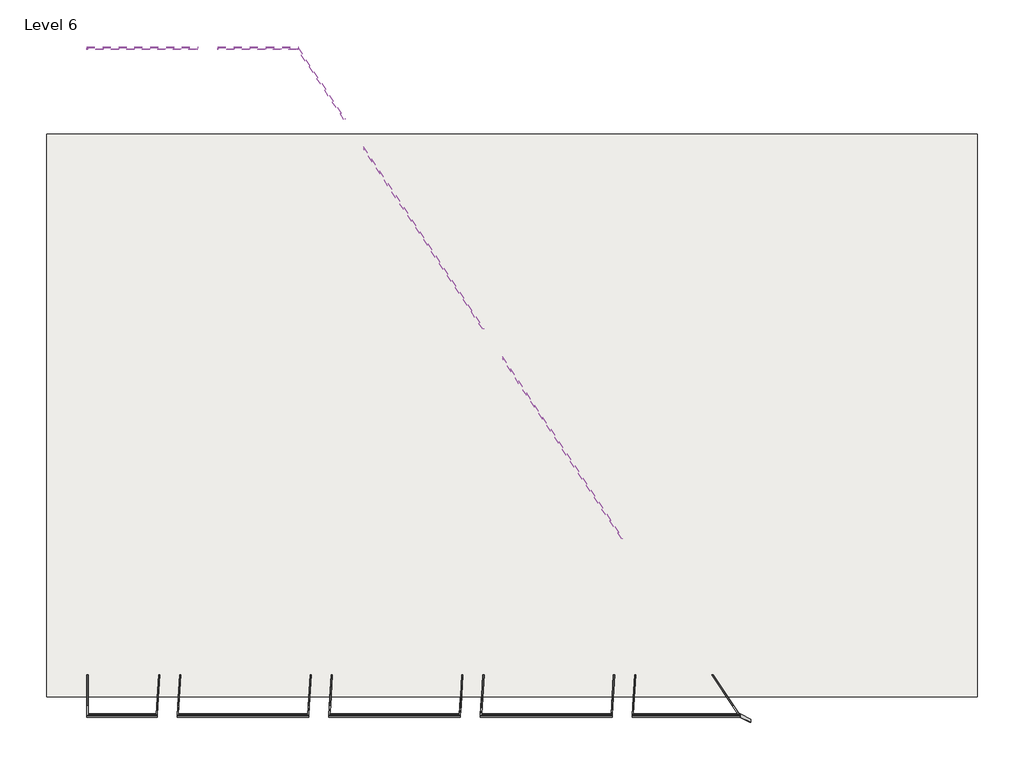
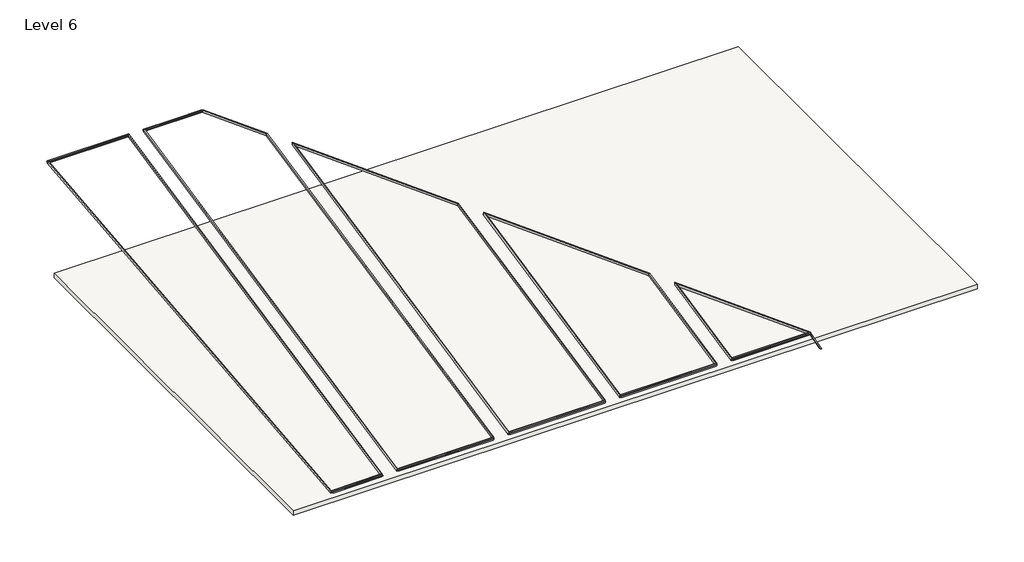
# One storey: 28 members, 1 slab.
"""IFC4 building model written with IfcOpenShell, lengths in millimetres."""

import ifcopenshell
import ifcopenshell.guid

model = None  # the IFC model being written
_history = None  # IfcOwnerHistory: only IFC2X3 demands one
_inside = {}  # id of a spatial element -> (the spatial element, [elements in it])
_under = {}  # id of a project, library or spatial element -> (it, [spatial elements below it])
_declared = {}  # id of a project -> (the project, [libraries it declares])
_typed = {}  # id of a type object -> (the type object, [elements of that type])
_made_of = {}  # id of a material, layer set ... -> (it, [elements and type objects made of it])


def new_model(schema):
    """Start an empty IFC model of exactly this schema.

    Asked for "IFC4X3", IfcOpenShell would pick the latest addendum, in which some entities
    have other attributes; the version numbers below select the first issue.
    IFC2X3 requires an IfcOwnerHistory on every rooted entity: one is made here for all.
    """
    global model, _history
    if schema == "IFC4X3":
        model = ifcopenshell.file(schema_version=(4, 3, 0, 0))
    else:
        model = ifcopenshell.file(schema=schema)
    _inside.clear()
    _under.clear()
    _declared.clear()
    _typed.clear()
    _made_of.clear()
    _history = None
    if model.schema == "IFC2X3":
        org = make("IfcOrganization", Name="unknown")
        user = make(
            "IfcPersonAndOrganization",
            ThePerson=make("IfcPerson", FamilyName="unknown"),
            TheOrganization=org,
        )
        app = make(
            "IfcApplication",
            ApplicationDeveloper=org,
            Version="unknown",
            ApplicationFullName="unknown",
            ApplicationIdentifier="unknown",
        )
        _history = make(
            "IfcOwnerHistory",
            OwningUser=user,
            OwningApplication=app,
            ChangeAction="ADDED",
            CreationDate=0,
        )
    return model


def make(cls, **values):
    """One entity of the class cls with the attributes given. An attribute that is None is left unset."""
    return model.create_entity(
        cls, **{name: value for name, value in values.items() if value is not None}
    )


def rooted(cls, **values):
    """An entity with a GlobalId (a new one), such as an element, a storey or a relation."""
    return make(cls, GlobalId=ifcopenshell.guid.new(), OwnerHistory=_history, **values)


def si_unit(unit_type, name, prefix=None):
    """IfcSIUnit, for example si_unit("LENGTHUNIT", "METRE", prefix="MILLI")."""
    return make("IfcSIUnit", UnitType=unit_type, Prefix=prefix, Name=name)


def assignment(units):
    """IfcUnitAssignment: the units of a project."""
    return None if units is None else make("IfcUnitAssignment", Units=units)


def point(xyz):
    """IfcCartesianPoint."""
    return None if xyz is None else make("IfcCartesianPoint", Coordinates=xyz)


def direction(xyz):
    """IfcDirection."""
    return None if xyz is None else make("IfcDirection", DirectionRatios=xyz)


def frame(location, z_axis=None, x_axis=None):
    """IfcAxis2Placement3D, a coordinate frame: its origin and axes. An axis left out is left unset."""
    return make(
        "IfcAxis2Placement3D",
        Location=point(location),
        Axis=direction(z_axis),
        RefDirection=direction(x_axis),
    )


def origin():
    """The frame at (0, 0, 0) with its axes left unset."""
    return frame((0.0, 0.0, 0.0))


def place(relative_to, where):
    """IfcLocalPlacement: puts the frame where relative to a parent placement (None: the world)."""
    return make(
        "IfcLocalPlacement", PlacementRelTo=relative_to, RelativePlacement=where
    )


def context(
    kind, dimensions, precision=None, world=None, true_north=None, identifier=None
):
    """IfcGeometricRepresentationContext, for example the 3D "Model" context."""
    return make(
        "IfcGeometricRepresentationContext",
        ContextIdentifier=identifier,
        ContextType=kind,
        CoordinateSpaceDimension=dimensions,
        Precision=precision,
        WorldCoordinateSystem=world,
        TrueNorth=true_north,
    )


def project(units=None, contexts=None):
    """IfcProject with its units and contexts."""
    return rooted(
        "IfcProject",
        Name="project",
        RepresentationContexts=contexts,
        UnitsInContext=assignment(units),
    )


def spatial(cls, under=None, at=None, **own):
    """A site, building, storey or space (cls), placed at a placement, below another one or the project."""
    s = rooted(cls, ObjectPlacement=at, **own)
    if under is not None:
        _under.setdefault(under.id(), (under, []))[1].append(s)
    return s


def polyline(points):
    """IfcPolyline through the points."""
    return make("IfcPolyline", Points=[point(p) for p in points])


def outline(outer, holes=None, kind="AREA"):
    """IfcArbitraryClosedProfileDef: a profile drawn as a closed curve; with holes, ...WithVoids."""
    if holes is None:
        return make("IfcArbitraryClosedProfileDef", ProfileType=kind, OuterCurve=outer)
    return make(
        "IfcArbitraryProfileDefWithVoids",
        ProfileType=kind,
        OuterCurve=outer,
        InnerCurves=holes,
    )


def extrude(swept, where, along, depth):
    """IfcExtrudedAreaSolid: the profile swept, set in the frame where, extruded along a direction by depth."""
    return make(
        "IfcExtrudedAreaSolid",
        SweptArea=swept,
        Position=where,
        ExtrudedDirection=direction(along),
        Depth=depth,
    )


def shape(context_of_items, identifier, shape_type, items):
    """IfcShapeRepresentation: the items that make up one representation, for example the "Body"."""
    return make(
        "IfcShapeRepresentation",
        ContextOfItems=context_of_items,
        RepresentationIdentifier=identifier,
        RepresentationType=shape_type,
        Items=items,
    )


def source(mapping_origin, context_of_items, identifier, shape_type, items):
    """IfcRepresentationMap: a shape defined once, which mapped items show again and again."""
    return make(
        "IfcRepresentationMap",
        MappingOrigin=mapping_origin,
        MappedRepresentation=shape(context_of_items, identifier, shape_type, items),
    )


def transform(
    local_origin,
    x_axis=None,
    y_axis=None,
    z_axis=None,
    scale=None,
    scale2=None,
    scale3=None,
    uniform=True,
):
    """IfcCartesianTransformationOperator3D, or its non-uniform kind. x_axis, y_axis, z_axis: its Axis1, 2, 3."""
    if uniform:
        return make(
            "IfcCartesianTransformationOperator3D",
            Axis1=direction(x_axis),
            Axis2=direction(y_axis),
            LocalOrigin=point(local_origin),
            Scale=scale,
            Axis3=direction(z_axis),
        )
    return make(
        "IfcCartesianTransformationOperator3DnonUniform",
        Axis1=direction(x_axis),
        Axis2=direction(y_axis),
        LocalOrigin=point(local_origin),
        Scale=scale,
        Axis3=direction(z_axis),
        Scale2=scale2,
        Scale3=scale3,
    )


def mapped(mapping_source, mapping_target):
    """IfcMappedItem: shows the shape of a source again, moved by a transform."""
    return make(
        "IfcMappedItem", MappingSource=mapping_source, MappingTarget=mapping_target
    )


def made_of(thing, what):
    """Note that an element or type object is made of a material, layer set ...; save() writes the relation."""
    if what is not None:
        _made_of.setdefault(what.id(), (what, []))[1].append(thing)
    return thing


def element(
    cls,
    number,
    at=None,
    inside=None,
    cuts=None,
    type_object=None,
    material=None,
    context=None,
    identifier="Body",
    shape_type=None,
    held_by="IfcProductDefinitionShape",
    body=None,
    shapes=None,
    **own,
):
    """One element of the class cls, such as IfcWall. Its Tag is "e" and its number.

    at: its placement. inside: the storey or other place that contains it. cuts: it is an
    opening in that element (IfcRelVoidsElement). A single representation is given by context,
    identifier, shape_type and body (its items); several are given by shapes. held_by: the class
    of the entity that holds the representations. save() writes the other relations.
    """
    e = rooted(cls, Tag="e%d" % number, ObjectPlacement=at, **own)
    if body is not None:
        shapes = [shape(context, identifier, shape_type, body)]
    if shapes is not None:
        e.Representation = make(held_by, Representations=shapes)
    if inside is not None:
        _inside.setdefault(inside.id(), (inside, []))[1].append(e)
    if cuts is not None:
        rooted(
            "IfcRelVoidsElement", RelatingBuildingElement=cuts, RelatedOpeningElement=e
        )
    if type_object is not None:
        _typed.setdefault(type_object.id(), (type_object, []))[1].append(e)
    return made_of(e, material)


def aggregate(whole, parts):
    """IfcRelAggregates: a whole, such as a stair, and the parts it consists of."""
    return rooted("IfcRelAggregates", RelatingObject=whole, RelatedObjects=parts)


def save(model, path):
    """Write the relations noted so far, then the file.

    IfcRelAggregates (storeys below a building ...), IfcRelContainedInSpatialStructure (elements
    in a storey), IfcRelDefinesByType, IfcRelAssociatesMaterial and IfcRelDeclares: one each for
    every whole, place, type object, material and project.
    """
    for whole, parts in _under.values():
        aggregate(whole, parts)
    for where, things in _inside.values():
        rooted(
            "IfcRelContainedInSpatialStructure",
            RelatedElements=things,
            RelatingStructure=where,
        )
    for kind, things in _typed.values():
        rooted("IfcRelDefinesByType", RelatedObjects=things, RelatingType=kind)
    for what, things in _made_of.values():
        rooted("IfcRelAssociatesMaterial", RelatedObjects=things, RelatingMaterial=what)
    for by, libraries in _declared.values():
        rooted("IfcRelDeclares", RelatingContext=by, RelatedDefinitions=libraries)
    model.write(path)


def rectangular_mullion_50_x_150mm_a1f019ed(model_context):
    return source(origin(), model_context, "Body", "SweptSolid", [
        extrude(outline(polyline([(0.0, 0.0), (-58.5251446, -50.0), (-1143.6098029, -50.0), (-1169.4475431, 0.0), (0.0, 0.0)])), frame((0.0, -75.0, 0.0), z_axis=(0.0, 1.0, 0.0), x_axis=(0.0, 0.0, 1.0)), (0.0, 0.0, 1.0), 150.0),
    ])


def rectangular_mullion_50_x_150mm_835307d9(model_context):
    return source(origin(), model_context, "Body", "SweptSolid", [
        extrude(outline(polyline([(0.0, 0.0), (-53.1084457, -50.0), (-6798.2667293, -50.0), (-6948.5596255, 0.0), (0.0, 0.0)])), frame((0.0, -75.0, 0.0), z_axis=(0.0, 1.0, 0.0), x_axis=(0.0, 0.0, 1.0)), (0.0, 0.0, 1.0), 150.0),
    ])


def rectangular_mullion_50_x_150mm_3a89df96(model_context):
    return source(origin(), model_context, "Body", "SweptSolid", [
        extrude(outline(polyline([(0.0, 0.0), (-50.0, -50.0), (-30950.0, -50.0), (-31000.0, 0.0), (0.0, 0.0)])), frame((0.0, -75.0, 0.0), z_axis=(0.0, 1.0, 0.0), x_axis=(0.0, 0.0, 1.0)), (0.0, 0.0, 1.0), 150.0),
    ])


def rectangular_mullion_50_x_150mm_0c0d54b6(model_context):
    return source(origin(), model_context, "Body", "SweptSolid", [
        extrude(outline(polyline([(0.0, 0.0), (-53.1084457, -50.0), (-31009.3272322, -50.0), (-31056.4007243, 0.0), (0.0, 0.0)])), frame((0.0, -75.0, 0.0), z_axis=(0.0, 1.0, 0.0), x_axis=(0.0, 0.0, 1.0)), (0.0, 0.0, 1.0), 150.0),
    ])


def rectangular_mullion_50_x_150mm_d5752ba3(model_context):
    return source(origin(), model_context, "Body", "SweptSolid", [
        extrude(outline(polyline([(0.0, 0.0), (-53.1084457, -50.0), (-26319.8624924, -50.0), (-26470.1553886, 0.0), (0.0, 0.0)])), frame((0.0, -75.0, 0.0), z_axis=(0.0, 1.0, 0.0), x_axis=(0.0, 0.0, 1.0)), (0.0, 0.0, 1.0), 150.0),
    ])


def rectangular_mullion_50_x_150mm_d02c79f9(model_context):
    return source(origin(), model_context, "Body", "SweptSolid", [
        extrude(outline(polyline([(0.0, 0.0), (-53.1084457, -50.0), (-16559.0646109, -50.0), (-16709.3575071, 0.0), (0.0, 0.0)])), frame((0.0, -75.0, 0.0), z_axis=(0.0, 1.0, 0.0), x_axis=(0.0, 0.0, 1.0)), (0.0, 0.0, 1.0), 150.0),
    ])


def rectangular_mullion_50_x_150mm_9a9dcb3f(model_context):
    return source(origin(), model_context, "Body", "SweptSolid", [
        extrude(outline(polyline([(0.0, 0.0), (-150.2928962, -50.0), (-8210.4264863, -50.0), (-8303.1882256, 0.0), (0.0, 0.0)])), frame((0.0, -75.0, 0.0), z_axis=(0.0, 1.0, 0.0), x_axis=(0.0, 0.0, 1.0)), (0.0, 0.0, 1.0), 150.0),
    ])


def rectangular_mullion_50_x_150mm_8c2aeeaa(model_context):
    return source(origin(), model_context, "Body", "SweptSolid", [
        extrude(outline(polyline([(0.0, 0.0), (-26.9507667, -50.0), (-3926.5430895, -50.0), (-3943.1772756, 0.0), (0.0, 0.0)])), frame((0.0, -75.0, 0.0), z_axis=(0.0, 1.0, 0.0), x_axis=(0.0, 0.0, 1.0)), (0.0, 0.0, 1.0), 150.0),
    ])


def rectangular_mullion_50_x_150mm_b203450d(model_context):
    return source(origin(), model_context, "Body", "SweptSolid", [
        extrude(outline(polyline([(0.0, 0.0), (-16.6341861, -50.0), (-27709.4619673, -50.0), (-27756.5354594, 0.0), (0.0, 0.0)])), frame((0.0, -75.0, 0.0), z_axis=(0.0, 1.0, 0.0), x_axis=(0.0, 0.0, 1.0)), (0.0, 0.0, 1.0), 150.0),
    ])


def rectangular_mullion_50_x_150mm_36cf8f86(model_context):
    return source(origin(), model_context, "Body", "SweptSolid", [
        extrude(outline(polyline([(0.0, 0.0), (-150.2928962, -50.0), (-10109.8797934, -50.0), (-10126.5139795, 0.0), (0.0, 0.0)])), frame((0.0, -75.0, 0.0), z_axis=(0.0, 1.0, 0.0), x_axis=(0.0, 0.0, 1.0)), (0.0, 0.0, 1.0), 150.0),
    ])


def rectangular_mullion_50_x_150mm_3d894c4c(model_context):
    return source(origin(), model_context, "Body", "SweptSolid", [
        extrude(outline(polyline([(0.0, 0.0), (-16.6341861, -50.0), (-17948.6640858, -50.0), (-17995.7375779, 0.0), (0.0, 0.0)])), frame((0.0, -75.0, 0.0), z_axis=(0.0, 1.0, 0.0), x_axis=(0.0, 0.0, 1.0)), (0.0, 0.0, 1.0), 150.0),
    ])


def rectangular_mullion_50_x_150mm_f4970be0(model_context):
    return source(origin(), model_context, "Body", "SweptSolid", [
        extrude(outline(polyline([(0.0, 0.0), (-16.6341861, -50.0), (-8187.8662042, -50.0), (-8234.9396963, 0.0), (0.0, 0.0)])), frame((0.0, -75.0, 0.0), z_axis=(0.0, 1.0, 0.0), x_axis=(0.0, 0.0, 1.0)), (0.0, 0.0, 1.0), 150.0),
    ])


def rectangular_mullion_50_x_150mm_5700b0c8(model_context):
    return source(origin(), model_context, "Body", "SweptSolid", [
        extrude(outline(polyline([(0.0, 0.0), (-86.4378444, -50.0), (-5081.8724884, -50.0), (-5115.611673, 0.0), (0.0, 0.0)])), frame((0.0, -75.0, 0.0), z_axis=(0.0, 1.0, 0.0), x_axis=(0.0, 0.0, 1.0)), (0.0, 0.0, 1.0), 150.0),
    ])


def rectangular_mullion_50_x_150mm_c12f4f4b(model_context):
    return source(origin(), model_context, "Body", "SweptSolid", [
        extrude(outline(polyline([(0.0, 0.0), (-98.1080667, -50.0), (-3682.0310611, -50.0), (-3710.9535778, 0.0), (0.0, 0.0)])), frame((0.0, -75.0, 0.0), z_axis=(0.0, 1.0, 0.0), x_axis=(0.0, 0.0, 1.0)), (0.0, 0.0, 1.0), 150.0),
    ])


def rectangular_mullion_50_x_150mm_5a0cd9cb(model_context):
    return source(origin(), model_context, "Body", "SweptSolid", [
        extrude(outline(polyline([(0.0, 0.0), (-92.7617394, -50.0), (-4930.0822697, -50.0), (-4983.1907154, 0.0), (0.0, 0.0)])), frame((0.0, -75.0, 0.0), z_axis=(0.0, 1.0, 0.0), x_axis=(0.0, 0.0, 1.0)), (0.0, 0.0, 1.0), 150.0),
    ])


def rectangular_mullion_50_x_150mm_5afc71bb(model_context):
    return source(origin(), model_context, "Body", "SweptSolid", [
        extrude(outline(polyline([(0.0, 0.0), (-47.0734921, -50.0), (-3194.7760444, -50.0), (-3244.7760444, 0.0), (0.0, 0.0)])), frame((0.0, -75.0, 0.0), z_axis=(0.0, 1.0, 0.0), x_axis=(0.0, 0.0, 1.0)), (0.0, 0.0, 1.0), 150.0),
    ])


def rectangular_mullion_50_x_150mm_f23ada83(model_context):
    return source(origin(), model_context, "Body", "SweptSolid", [
        extrude(outline(polyline([(0.0, 0.0), (-47.0734921, -50.0), (-6024.3583142, -50.0), (-6077.4667599, 0.0), (0.0, 0.0)])), frame((0.0, -75.0, 0.0), z_axis=(0.0, 1.0, 0.0), x_axis=(0.0, 0.0, 1.0)), (0.0, 0.0, 1.0), 150.0),
    ])


def rectangular_mullion_50_x_150mm_0be3d6d3(model_context):
    return source(origin(), model_context, "Body", "SweptSolid", [
        extrude(outline(polyline([(0.0, 0.0), (-50.0, -50.0), (-5062.5032273, -50.0), (-5115.611673, 0.0), (0.0, 0.0)])), frame((0.0, -75.0, 0.0), z_axis=(0.0, 1.0, 0.0), x_axis=(0.0, 0.0, 1.0)), (0.0, 0.0, 1.0), 150.0),
    ])


def rectangular_mullion_50_x_150mm_139992b9(model_context):
    return source(origin(), model_context, "Body", "SweptSolid", [
        extrude(outline(polyline([(0.0, 0.0), (-47.0734921, -50.0), (-3684.0028111, -50.0), (-3710.9535778, 0.0), (0.0, 0.0)])), frame((0.0, -75.0, 0.0), z_axis=(0.0, 1.0, 0.0), x_axis=(0.0, 0.0, 1.0)), (0.0, 0.0, 1.0), 150.0),
    ])


def rectangular_mullion_50_x_150mm_45cfd48e(model_context):
    return source(origin(), model_context, "Body", "SweptSolid", [
        extrude(outline(polyline([(0.0, 0.0), (-108.6604448, -50.0), (-3159.4549255, -50.0), (-3244.7760444, 0.0), (0.0, 0.0)])), frame((0.0, -75.0, 0.0), z_axis=(0.0, 1.0, 0.0), x_axis=(0.0, 0.0, 1.0)), (0.0, 0.0, 1.0), 150.0),
    ])


def rectangular_mullion_50_x_150mm_f412d67c(model_context):
    return source(origin(), model_context, "Body", "SweptSolid", [
        extrude(outline(polyline([(0.0, 0.0), (-29.3010691, -50.0), (-5992.1456409, -50.0), (-6077.4667599, 0.0), (0.0, 0.0)])), frame((0.0, -75.0, 0.0), z_axis=(0.0, 1.0, 0.0), x_axis=(0.0, 0.0, 1.0)), (0.0, 0.0, 1.0), 150.0),
    ])


def rectangular_mullion_50_x_150mm_460fb724(model_context):
    return source(origin(), model_context, "Body", "SweptSolid", [
        extrude(outline(polyline([(0.0, 0.0), (-29.3010691, -50.0), (-4821.4590794, -50.0), (-4983.1907154, 0.0), (0.0, 0.0)])), frame((0.0, -75.0, 0.0), z_axis=(0.0, 1.0, 0.0), x_axis=(0.0, 0.0, 1.0)), (0.0, 0.0, 1.0), 150.0),
    ])


model = new_model("IFC4")

# Units and contexts
model_context = context("Model", 3, world=origin())
ifc_project = project(units=[si_unit("LENGTHUNIT", "METRE", prefix="MILLI")], contexts=[model_context])

# Site, building, storey
site = spatial("IfcSite", under=ifc_project)
building = spatial("IfcBuilding", under=site)
storey = spatial("IfcBuildingStorey", under=building, Name="Level 6", Elevation=15000.0)

# Members
placement = place(None, origin())
rectangular_mullion_50_x_150mm_shape = rectangular_mullion_50_x_150mm_a1f019ed(model_context)
element("IfcMember", 1, ObjectType="Rectangular Mullion : 50 x 150mm", at=placement, inside=storey, context=model_context, shape_type="MappedRepresentation", body=[
    mapped(rectangular_mullion_50_x_150mm_shape, transform((25283.6081085, -10856.2576342, 16077.9460567), x_axis=(0.9035184763618896, 0.10483186655429763, 0.41552935230550386), y_axis=(-0.004309282844983733, 0.9717923608297843, -0.23579872246099295), z_axis=(-0.42852747047774137, 0.2112578689365591, 0.8784841033612003))),
])
rectangular_mullion_50_x_150mm_2_shape = rectangular_mullion_50_x_150mm_835307d9(model_context)
element("IfcMember", 2, ObjectType="Rectangular Mullion : 50 x 150mm", at=placement, inside=storey, context=model_context, shape_type="MappedRepresentation", body=[
    mapped(rectangular_mullion_50_x_150mm_2_shape, transform((20300.417393, -10856.2576342, 16077.9460567), x_axis=(-0.9981839259219352, 0.05990993649800364, 0.006296788060437585), y_axis=(0.0, 0.10452846326765378, -0.9945218953682734), z_axis=(-0.06023993717686712, -0.9927157699340269, -0.10433863183509343))),
])
rectangular_mullion_50_x_150mm_3_shape = rectangular_mullion_50_x_150mm_3a89df96(model_context)
element("IfcMember", 3, ObjectType="Rectangular Mullion : 50 x 150mm", at=placement, inside=storey, context=model_context, shape_type="MappedRepresentation", body=[
    mapped(rectangular_mullion_50_x_150mm_3_shape, transform((-4866.8918915, -10856.2576342, 16077.9460567), x_axis=(-1.0, 0.0, 0.0), y_axis=(0.0, 0.10452846326765393, -0.9945218953682733), z_axis=(0.0, -0.9945218953682733, -0.10452846326765393))),
])
rectangular_mullion_50_x_150mm_4_shape = rectangular_mullion_50_x_150mm_0c0d54b6(model_context)
element("IfcMember", 4, ObjectType="Rectangular Mullion : 50 x 150mm", at=placement, inside=storey, context=model_context, shape_type="MappedRepresentation", body=[
    mapped(rectangular_mullion_50_x_150mm_4_shape, transform((-699.582607, -10856.2576342, 16077.9460567), x_axis=(-0.998183925921935, 0.05990993649800494, 0.00629678806043772), y_axis=(0.0, 0.10452846326765394, -0.9945218953682733), z_axis=(-0.06023993717686844, -0.9927157699340269, -0.1043386318350936))),
])
rectangular_mullion_50_x_150mm_5_shape = rectangular_mullion_50_x_150mm_d5752ba3(model_context)
element("IfcMember", 5, ObjectType="Rectangular Mullion : 50 x 150mm", at=placement, inside=storey, context=model_context, shape_type="MappedRepresentation", body=[
    mapped(rectangular_mullion_50_x_150mm_5_shape, transform((6300.417393, -10856.2576342, 16077.9460567), x_axis=(-0.9981839259219351, 0.059909936498005, 0.006296788060437727), y_axis=(0.0, 0.10452846326765393, -0.9945218953682734), z_axis=(-0.060239937176868485, -0.9927157699340268, -0.10433863183509358))),
])
rectangular_mullion_50_x_150mm_6_shape = rectangular_mullion_50_x_150mm_d02c79f9(model_context)
element("IfcMember", 6, ObjectType="Rectangular Mullion : 50 x 150mm", at=placement, inside=storey, context=model_context, shape_type="MappedRepresentation", body=[
    mapped(rectangular_mullion_50_x_150mm_6_shape, transform((13300.417393, -10856.2576342, 16077.9460567), x_axis=(-0.998183925921935, 0.05990993649800466, 0.006296788060437691), y_axis=(0.0, 0.1045284632676539, -0.9945218953682733), z_axis=(-0.06023993717686815, -0.9927157699340269, -0.10433863183509358))),
])
rectangular_mullion_50_x_150mm_7_shape = rectangular_mullion_50_x_150mm_9a9dcb3f(model_context)
element("IfcMember", 7, ObjectType="Rectangular Mullion : 50 x 150mm", at=placement, inside=storey, context=model_context, shape_type="MappedRepresentation", body=[
    mapped(rectangular_mullion_50_x_150mm_7_shape, transform((20718.9981883, -3958.3129157, 16802.9492613), x_axis=(0.83533461340766, 0.5467302903451189, 0.05746366906330552), y_axis=(0.0, 0.10452846326765378, -0.9945218953682733), z_axis=(-0.5497418336301824, 0.83075856299291, 0.08731624345378214))),
])
element("IfcMember", 8, ObjectType="Rectangular Mullion : 50 x 150mm", at=placement, inside=storey, context=model_context, shape_type="MappedRepresentation", body=[
    mapped(rectangular_mullion_50_x_150mm_4_shape, transform((248.7197815, 19973.9211222, 19318.328418), x_axis=(0.998183925921935, -0.05990993649800525, -0.006296788060437753), y_axis=(0.0, 0.10452846326765385, -0.9945218953682734), z_axis=(0.06023993717686875, 0.9927157699340269, 0.10433863183509351))),
])
rectangular_mullion_50_x_150mm_8_shape = rectangular_mullion_50_x_150mm_8c2aeeaa(model_context)
element("IfcMember", 9, ObjectType="Rectangular Mullion : 50 x 150mm", at=placement, inside=storey, context=model_context, shape_type="MappedRepresentation", body=[
    mapped(rectangular_mullion_50_x_150mm_8_shape, transform((4882.2065994, 19973.9211222, 19318.328418), x_axis=(0.8353346134076604, 0.5467302903451184, 0.05746366906330546), y_axis=(0.0, 0.10452846326765367, -0.9945218953682733), z_axis=(-0.5497418336301818, 0.8307585629929103, 0.08731624345378203))),
])
rectangular_mullion_50_x_150mm_9_shape = rectangular_mullion_50_x_150mm_b203450d(model_context)
element("IfcMember", 10, ObjectType="Rectangular Mullion : 50 x 150mm", at=placement, inside=storey, context=model_context, shape_type="MappedRepresentation", body=[
    mapped(rectangular_mullion_50_x_150mm_9_shape, transform((7049.9361052, 16698.0928351, 18974.024991), x_axis=(0.998183925921935, -0.05990993649800497, -0.006296788060437724), y_axis=(0.0, 0.10452846326765391, -0.9945218953682734), z_axis=(0.060239937176868465, 0.9927157699340269, 0.10433863183509358))),
])
rectangular_mullion_50_x_150mm_10_shape = rectangular_mullion_50_x_150mm_36cf8f86(model_context)
element("IfcMember", 11, ObjectType="Rectangular Mullion : 50 x 150mm", at=placement, inside=storey, context=model_context, shape_type="MappedRepresentation", body=[
    mapped(rectangular_mullion_50_x_150mm_10_shape, transform((7894.9778907, 15421.0830526, 18839.8058544), x_axis=(0.83533461340766, 0.546730290345119, 0.05746366906330553), y_axis=(0.0, 0.10452846326765391, -0.9945218953682733), z_axis=(-0.5497418336301826, 0.83075856299291, 0.0873162434537823))),
])
rectangular_mullion_50_x_150mm_11_shape = rectangular_mullion_50_x_150mm_3d894c4c(model_context)
element("IfcMember", 12, ObjectType="Rectangular Mullion : 50 x 150mm", at=placement, inside=storey, context=model_context, shape_type="MappedRepresentation", body=[
    mapped(rectangular_mullion_50_x_150mm_11_shape, transform((13461.946254, 7008.3948509, 17955.5966945), x_axis=(0.9981839259219351, -0.05990993649800527, -0.006296788060437756), y_axis=(0.0, 0.10452846326765394, -0.9945218953682734), z_axis=(0.060239937176868756, 0.9927157699340268, 0.10433863183509359))),
])
element("IfcMember", 13, ObjectType="Rectangular Mullion : 50 x 150mm", at=placement, inside=storey, context=model_context, shape_type="MappedRepresentation", body=[
    mapped(rectangular_mullion_50_x_150mm_10_shape, transform((14306.9880395, 5731.3850685, 17821.3775579), x_axis=(0.8353346134076599, 0.5467302903451192, 0.05746366906330556), y_axis=(0.0, 0.10452846326765397, -0.9945218953682733), z_axis=(-0.5497418336301827, 0.8307585629929097, 0.08731624345378232))),
])
rectangular_mullion_50_x_150mm_12_shape = rectangular_mullion_50_x_150mm_f4970be0(model_context)
element("IfcMember", 14, ObjectType="Rectangular Mullion : 50 x 150mm", at=placement, inside=storey, context=model_context, shape_type="MappedRepresentation", body=[
    mapped(rectangular_mullion_50_x_150mm_12_shape, transform((19873.9564029, -2681.3031332, 16937.1683979), x_axis=(0.9981839259219351, -0.05990993649800277, -0.006296788060437492), y_axis=(0.0, 0.10452846326765383, -0.9945218953682733), z_axis=(0.06023993717686625, 0.992715769934027, 0.10433863183509351))),
])
rectangular_mullion_50_x_150mm_13_shape = rectangular_mullion_50_x_150mm_5700b0c8(model_context)
element("IfcMember", 15, ObjectType="Rectangular Mullion : 50 x 150mm", at=placement, inside=storey, context=model_context, shape_type="MappedRepresentation", body=[
    mapped(rectangular_mullion_50_x_150mm_13_shape, transform((248.7197815, 19973.9211222, 19318.328418), x_axis=(0.0, 0.08715574274766863, 0.9961946980917447), y_axis=(0.0, -0.9961946980917447, 0.08715574274766863), z_axis=(1.0, 0.0, 0.0))),
])
rectangular_mullion_50_x_150mm_14_shape = rectangular_mullion_50_x_150mm_c12f4f4b(model_context)
element("IfcMember", 16, ObjectType="Rectangular Mullion : 50 x 150mm", at=placement, inside=storey, context=model_context, shape_type="MappedRepresentation", body=[
    mapped(rectangular_mullion_50_x_150mm_14_shape, transform((4882.2065994, 19973.9211222, 19318.328418), x_axis=(0.0, 0.08715574274766863, 0.9961946980917447), y_axis=(0.0, -0.9961946980917447, 0.08715574274766863), z_axis=(1.0, 0.0, 0.0))),
])
rectangular_mullion_50_x_150mm_15_shape = rectangular_mullion_50_x_150mm_5a0cd9cb(model_context)
element("IfcMember", 17, ObjectType="Rectangular Mullion : 50 x 150mm", at=placement, inside=storey, context=model_context, shape_type="MappedRepresentation", body=[
    mapped(rectangular_mullion_50_x_150mm_15_shape, transform((25283.6081085, -10856.2576342, 16077.9460567), x_axis=(0.0, -0.9945218953682733, -0.10452846326765391), y_axis=(0.0, 0.10452846326765391, -0.9945218953682733), z_axis=(1.0, 0.0, 0.0))),
])
rectangular_mullion_50_x_150mm_16_shape = rectangular_mullion_50_x_150mm_5afc71bb(model_context)
element("IfcMember", 18, ObjectType="Rectangular Mullion : 50 x 150mm", at=placement, inside=storey, context=model_context, shape_type="MappedRepresentation", body=[
    mapped(rectangular_mullion_50_x_150mm_16_shape, transform((-1622.1158471, -10856.2576342, 16077.9460567), x_axis=(0.0, -0.9945218953682733, -0.10452846326765391), y_axis=(0.0, 0.10452846326765391, -0.9945218953682733), z_axis=(1.0, 0.0, 0.0))),
])
rectangular_mullion_50_x_150mm_17_shape = rectangular_mullion_50_x_150mm_f23ada83(model_context)
element("IfcMember", 19, ObjectType="Rectangular Mullion : 50 x 150mm", at=placement, inside=storey, context=model_context, shape_type="MappedRepresentation", body=[
    mapped(rectangular_mullion_50_x_150mm_17_shape, transform((5377.8841529, -10856.2576342, 16077.9460567), x_axis=(0.0, -0.9945218953682733, -0.10452846326765391), y_axis=(0.0, 0.10452846326765391, -0.9945218953682733), z_axis=(1.0, 0.0, 0.0))),
])
element("IfcMember", 20, ObjectType="Rectangular Mullion : 50 x 150mm", at=placement, inside=storey, context=model_context, shape_type="MappedRepresentation", body=[
    mapped(rectangular_mullion_50_x_150mm_17_shape, transform((12377.8841529, -10856.2576342, 16077.9460567), x_axis=(0.0, -0.9945218953682733, -0.10452846326765391), y_axis=(0.0, 0.10452846326765391, -0.9945218953682733), z_axis=(1.0, 0.0, 0.0))),
])
element("IfcMember", 21, ObjectType="Rectangular Mullion : 50 x 150mm", at=placement, inside=storey, context=model_context, shape_type="MappedRepresentation", body=[
    mapped(rectangular_mullion_50_x_150mm_17_shape, transform((19377.8841529, -10856.2576342, 16077.9460567), x_axis=(0.0, -0.9945218953682733, -0.10452846326765391), y_axis=(0.0, 0.10452846326765391, -0.9945218953682733), z_axis=(1.0, 0.0, 0.0))),
])
rectangular_mullion_50_x_150mm_18_shape = rectangular_mullion_50_x_150mm_0be3d6d3(model_context)
element("IfcMember", 22, ObjectType="Rectangular Mullion : 50 x 150mm", at=placement, inside=storey, context=model_context, shape_type="MappedRepresentation", body=[
    mapped(rectangular_mullion_50_x_150mm_18_shape, transform((-4866.8918915, 19973.9211222, 19318.328418), x_axis=(0.0, 0.9945218953682733, 0.10452846326765391), y_axis=(0.0, 0.10452846326765391, -0.9945218953682733), z_axis=(-1.0, 0.0, 0.0))),
])
rectangular_mullion_50_x_150mm_19_shape = rectangular_mullion_50_x_150mm_139992b9(model_context)
element("IfcMember", 23, ObjectType="Rectangular Mullion : 50 x 150mm", at=placement, inside=storey, context=model_context, shape_type="MappedRepresentation", body=[
    mapped(rectangular_mullion_50_x_150mm_19_shape, transform((1171.2530216, 19973.9211222, 19318.328418), x_axis=(0.0, 0.9945218953682733, 0.10452846326765391), y_axis=(0.0, 0.10452846326765391, -0.9945218953682733), z_axis=(-1.0, 0.0, 0.0))),
])
rectangular_mullion_50_x_150mm_20_shape = rectangular_mullion_50_x_150mm_45cfd48e(model_context)
element("IfcMember", 24, ObjectType="Rectangular Mullion : 50 x 150mm", at=placement, inside=storey, context=model_context, shape_type="MappedRepresentation", body=[
    mapped(rectangular_mullion_50_x_150mm_20_shape, transform((-4866.8918915, -10856.2576342, 16077.9460567), x_axis=(0.0, 0.24192189559966848, 0.9702957262759964), y_axis=(0.0, 0.9702957262759964, -0.24192189559966848), z_axis=(-1.0, 0.0, 0.0))),
])
rectangular_mullion_50_x_150mm_21_shape = rectangular_mullion_50_x_150mm_f412d67c(model_context)
element("IfcMember", 25, ObjectType="Rectangular Mullion : 50 x 150mm", at=placement, inside=storey, context=model_context, shape_type="MappedRepresentation", body=[
    mapped(rectangular_mullion_50_x_150mm_21_shape, transform((-699.582607, -10856.2576342, 16077.9460567), x_axis=(0.0, 0.24192189559966848, 0.9702957262759964), y_axis=(0.0, 0.9702957262759964, -0.24192189559966848), z_axis=(-1.0, 0.0, 0.0))),
])
element("IfcMember", 26, ObjectType="Rectangular Mullion : 50 x 150mm", at=placement, inside=storey, context=model_context, shape_type="MappedRepresentation", body=[
    mapped(rectangular_mullion_50_x_150mm_21_shape, transform((6300.417393, -10856.2576342, 16077.9460567), x_axis=(0.0, 0.24192189559966848, 0.9702957262759964), y_axis=(0.0, 0.9702957262759964, -0.24192189559966848), z_axis=(-1.0, 0.0, 0.0))),
])
element("IfcMember", 27, ObjectType="Rectangular Mullion : 50 x 150mm", at=placement, inside=storey, context=model_context, shape_type="MappedRepresentation", body=[
    mapped(rectangular_mullion_50_x_150mm_21_shape, transform((13300.417393, -10856.2576342, 16077.9460567), x_axis=(0.0, 0.24192189559966848, 0.9702957262759964), y_axis=(0.0, 0.9702957262759964, -0.24192189559966848), z_axis=(-1.0, 0.0, 0.0))),
])
rectangular_mullion_50_x_150mm_22_shape = rectangular_mullion_50_x_150mm_460fb724(model_context)
element("IfcMember", 28, ObjectType="Rectangular Mullion : 50 x 150mm", at=placement, inside=storey, context=model_context, shape_type="MappedRepresentation", body=[
    mapped(rectangular_mullion_50_x_150mm_22_shape, transform((20300.417393, -10856.2576342, 16077.9460567), x_axis=(0.0, 0.24192189559966848, 0.9702957262759964), y_axis=(0.0, 0.9702957262759964, -0.24192189559966848), z_axis=(-1.0, 0.0, 0.0))),
])

# Slab
element("IfcSlab", 29, ObjectType="Generic 300mm", at=placement, inside=storey, context=model_context, shape_type="SweptSolid", body=[
    extrude(outline(polyline([(-6732.0028633, 15998.757723), (36243.4971367, 15998.757723), (36243.4971367, -10001.242277), (-6732.0028633, -10001.242277), (-6732.0028633, 15998.757723)])), frame((0.0, 0.0, 14700.0), z_axis=(0.0, 0.0, 1.0), x_axis=(1.0, 0.0, 0.0)), (0.0, 0.0, 1.0), 300.0),
])

save(model, "model.ifc")

# Revit data of these elements
# Type "Rectangular Mullion : 50 x 150mm"
#   built-in parameter 1007304 = 0.492126 (stored number, unit not read)
#   built-in parameter 1007301 = 0.082021 (stored number, unit not read)
#   built-in parameter 1007300 = 0.082021 (stored number, unit not read)
# Type "Generic 300mm"
#   Function = 0
#   Layers, outside or top first: 0.300 m no material (function 1)
# Elements 1, 2, 3, 4, 5, 6, 7, 8, 9, 10, 11, 12, 13, 14, 15, 16, 17, 18, 19, 20, 21, 22, 23, 24, 25, 26, 27, 28 (IfcMember, "Rectangular Mullion : 50 x 150mm")
#   Phase Created = New Construction
#   Materials on its faces: "Metal - Aluminium"
# Element 29 (IfcSlab, "Generic 300mm")
#   built-in parameter 1001955 = 3.14159 (stored number, unit not read)
#   Height Offset From Level = 0.000 m
#   Phase Created = New Construction
#   Materials on its faces: "Default Floor"
# Materials
#   "Metal - Aluminium": class "Metal", colour RGB 247 247 247, transparency 0
#   "Default Floor": class "Miscellaneous", colour RGB 127 127 127, transparency 0
